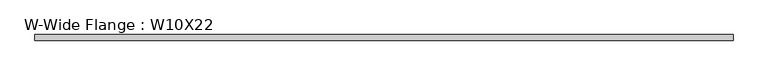
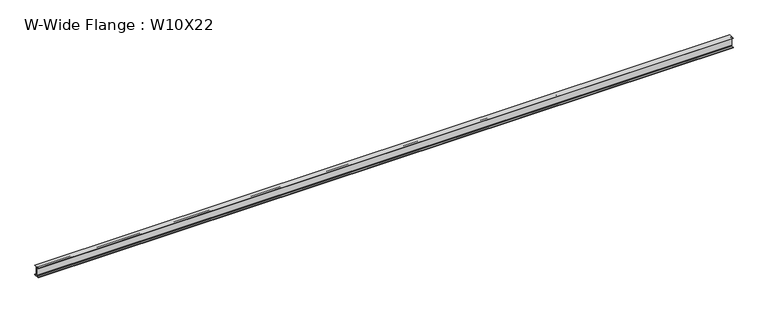
"""IFC4 building model written with IfcOpenShell, lengths in millimetres: beam geometry, W-Wide Flange : W10X22."""

from ifc_helpers import new_model, si_unit, point, frame, frame_2d, origin, place, context, project, spatial, polyline, circle_curve, trimmed, segment, composite_curve, outline, extrude, source, transform, mapped, element, save


def w_wide_flange_w10x22_977d26c2(model_context):
    return source(origin(), model_context, "Body", "SweptSolid", [
        extrude(outline(composite_curve([segment(polyline([(73.025, -120.396), (73.025, -129.54), (-73.025, -129.54), (-73.025, -120.396), (-17.7165, -120.396)]), True, "CONTINUOUS"), segment(trimmed(circle_curve(frame_2d((-17.7165, -105.7275)), 14.6685), [point((-17.7165, -120.396))], [point((-3.048, -105.7275))], True, "CARTESIAN"), True, "CONTINUOUS"), segment(polyline([(-3.048, -105.7275), (-3.048, 105.7275)]), True, "CONTINUOUS"), segment(trimmed(circle_curve(frame_2d((-17.7165, 105.7275)), 14.6685), [point((-3.048, 105.7275))], [point((-17.7165, 120.396))], True, "CARTESIAN"), True, "CONTINUOUS"), segment(polyline([(-17.7165, 120.396), (-73.025, 120.396), (-73.025, 129.54), (73.025, 129.54), (73.025, 120.396), (17.7165, 120.396)]), True, "CONTINUOUS"), segment(trimmed(circle_curve(frame_2d((17.7165, 105.7275)), 14.6685), [point((17.7165, 120.396))], [point((3.048, 105.7275))], True, "CARTESIAN"), True, "CONTINUOUS"), segment(polyline([(3.048, 105.7275), (3.048, -105.7275)]), True, "CONTINUOUS"), segment(trimmed(circle_curve(frame_2d((17.7165, -105.7275)), 14.6685), [point((3.048, -105.7275))], [point((17.7165, -120.396))], True, "CARTESIAN"), True, "CONTINUOUS"), segment(polyline([(17.7165, -120.396), (73.025, -120.396)]), True, "CONTINUOUS")], self_intersect=False)), frame((-8993.5510904, 0.0, 0.0), z_axis=(1.0, 0.0, 0.0), x_axis=(0.0, 1.0, 0.0)), (0.0, 0.0, 1.0), 17987.1021808),
    ])


if __name__ == "__main__":
    model = new_model("IFC4")
    model_context = context("Model", 3, world=origin())
    ifc_project = project(units=[si_unit("LENGTHUNIT", "METRE", prefix="MILLI")], contexts=[model_context])
    site = spatial("IfcSite", under=ifc_project)
    building = spatial("IfcBuilding", under=site)
    placement = place(None, origin())
    w_wide_flange_w10x22_shape = w_wide_flange_w10x22_977d26c2(model_context)
    element("IfcBeam", 1, ObjectType="W-Wide Flange : W10X22", at=placement, inside=building, context=model_context, shape_type="MappedRepresentation", body=[
        mapped(w_wide_flange_w10x22_shape, transform((0.0, 0.0, 0.0), x_axis=(1.0, 0.0, 0.0), y_axis=(0.0, 1.0, 0.0), z_axis=(0.0, 0.0, 1.0))),
    ])
    save(model, "model.ifc")

# Revit data of these elements
# Type "W-Wide Flange : W10X22"
#   Assembly Code = "B10"
#   W = 22
#   Length [instance default] = 5' - 0"
#   bf = 0' - 5 3/4"
#   d = 0' - 10.2"
#   k = 0' - 0 15/16"
#   k2 = 0' - 0.5775"
#   tf = 0' - 0.36"
#   tw = 0' - 0.24"
#   A = 0.0450694 SF
#   Structural Material [instance default] = Steel ASTM A992
# Element 1 (IfcBeam, "W-Wide Flange : W10X22")
#   Materials on its faces: "Steel ASTM A992"
# Materials
#   "Steel ASTM A992": class "Metal", colour RGB 199 199 199, transparency 0, Description = "Structural steel 50ksi", Cost = 0
